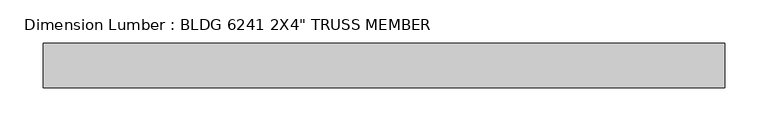
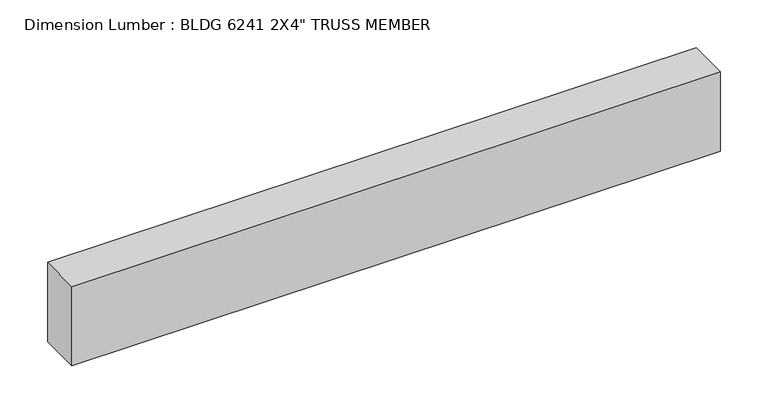
"""IFC4 building model written with IfcOpenShell, lengths in millimetres: beam geometry."""

import ifcopenshell
import ifcopenshell.guid

model = None  # the IFC model being written
_history = None  # IfcOwnerHistory: only IFC2X3 demands one
_inside = {}  # id of a spatial element -> (the spatial element, [elements in it])
_under = {}  # id of a project, library or spatial element -> (it, [spatial elements below it])
_declared = {}  # id of a project -> (the project, [libraries it declares])
_typed = {}  # id of a type object -> (the type object, [elements of that type])
_made_of = {}  # id of a material, layer set ... -> (it, [elements and type objects made of it])


def new_model(schema):
    """Start an empty IFC model of exactly this schema.

    Asked for "IFC4X3", IfcOpenShell would pick the latest addendum, in which some entities
    have other attributes; the version numbers below select the first issue.
    IFC2X3 requires an IfcOwnerHistory on every rooted entity: one is made here for all.
    """
    global model, _history
    if schema == "IFC4X3":
        model = ifcopenshell.file(schema_version=(4, 3, 0, 0))
    else:
        model = ifcopenshell.file(schema=schema)
    _inside.clear()
    _under.clear()
    _declared.clear()
    _typed.clear()
    _made_of.clear()
    _history = None
    if model.schema == "IFC2X3":
        org = make("IfcOrganization", Name="unknown")
        user = make(
            "IfcPersonAndOrganization",
            ThePerson=make("IfcPerson", FamilyName="unknown"),
            TheOrganization=org,
        )
        app = make(
            "IfcApplication",
            ApplicationDeveloper=org,
            Version="unknown",
            ApplicationFullName="unknown",
            ApplicationIdentifier="unknown",
        )
        _history = make(
            "IfcOwnerHistory",
            OwningUser=user,
            OwningApplication=app,
            ChangeAction="ADDED",
            CreationDate=0,
        )
    return model


def make(cls, **values):
    """One entity of the class cls with the attributes given. An attribute that is None is left unset."""
    return model.create_entity(
        cls, **{name: value for name, value in values.items() if value is not None}
    )


def rooted(cls, **values):
    """An entity with a GlobalId (a new one), such as an element, a storey or a relation."""
    return make(cls, GlobalId=ifcopenshell.guid.new(), OwnerHistory=_history, **values)


def si_unit(unit_type, name, prefix=None):
    """IfcSIUnit, for example si_unit("LENGTHUNIT", "METRE", prefix="MILLI")."""
    return make("IfcSIUnit", UnitType=unit_type, Prefix=prefix, Name=name)


def assignment(units):
    """IfcUnitAssignment: the units of a project."""
    return None if units is None else make("IfcUnitAssignment", Units=units)


def point(xyz):
    """IfcCartesianPoint."""
    return None if xyz is None else make("IfcCartesianPoint", Coordinates=xyz)


def direction(xyz):
    """IfcDirection."""
    return None if xyz is None else make("IfcDirection", DirectionRatios=xyz)


def frame(location, z_axis=None, x_axis=None):
    """IfcAxis2Placement3D, a coordinate frame: its origin and axes. An axis left out is left unset."""
    return make(
        "IfcAxis2Placement3D",
        Location=point(location),
        Axis=direction(z_axis),
        RefDirection=direction(x_axis),
    )


def origin():
    """The frame at (0, 0, 0) with its axes left unset."""
    return frame((0.0, 0.0, 0.0))


def place(relative_to, where):
    """IfcLocalPlacement: puts the frame where relative to a parent placement (None: the world)."""
    return make(
        "IfcLocalPlacement", PlacementRelTo=relative_to, RelativePlacement=where
    )


def context(
    kind, dimensions, precision=None, world=None, true_north=None, identifier=None
):
    """IfcGeometricRepresentationContext, for example the 3D "Model" context."""
    return make(
        "IfcGeometricRepresentationContext",
        ContextIdentifier=identifier,
        ContextType=kind,
        CoordinateSpaceDimension=dimensions,
        Precision=precision,
        WorldCoordinateSystem=world,
        TrueNorth=true_north,
    )


def project(units=None, contexts=None):
    """IfcProject with its units and contexts."""
    return rooted(
        "IfcProject",
        Name="project",
        RepresentationContexts=contexts,
        UnitsInContext=assignment(units),
    )


def spatial(cls, under=None, at=None, **own):
    """A site, building, storey or space (cls), placed at a placement, below another one or the project."""
    s = rooted(cls, ObjectPlacement=at, **own)
    if under is not None:
        _under.setdefault(under.id(), (under, []))[1].append(s)
    return s


def polyline(points):
    """IfcPolyline through the points."""
    return make("IfcPolyline", Points=[point(p) for p in points])


def outline(outer, holes=None, kind="AREA"):
    """IfcArbitraryClosedProfileDef: a profile drawn as a closed curve; with holes, ...WithVoids."""
    if holes is None:
        return make("IfcArbitraryClosedProfileDef", ProfileType=kind, OuterCurve=outer)
    return make(
        "IfcArbitraryProfileDefWithVoids",
        ProfileType=kind,
        OuterCurve=outer,
        InnerCurves=holes,
    )


def extrude(swept, where, along, depth):
    """IfcExtrudedAreaSolid: the profile swept, set in the frame where, extruded along a direction by depth."""
    return make(
        "IfcExtrudedAreaSolid",
        SweptArea=swept,
        Position=where,
        ExtrudedDirection=direction(along),
        Depth=depth,
    )


def shape(context_of_items, identifier, shape_type, items):
    """IfcShapeRepresentation: the items that make up one representation, for example the "Body"."""
    return make(
        "IfcShapeRepresentation",
        ContextOfItems=context_of_items,
        RepresentationIdentifier=identifier,
        RepresentationType=shape_type,
        Items=items,
    )


def source(mapping_origin, context_of_items, identifier, shape_type, items):
    """IfcRepresentationMap: a shape defined once, which mapped items show again and again."""
    return make(
        "IfcRepresentationMap",
        MappingOrigin=mapping_origin,
        MappedRepresentation=shape(context_of_items, identifier, shape_type, items),
    )


def transform(
    local_origin,
    x_axis=None,
    y_axis=None,
    z_axis=None,
    scale=None,
    scale2=None,
    scale3=None,
    uniform=True,
):
    """IfcCartesianTransformationOperator3D, or its non-uniform kind. x_axis, y_axis, z_axis: its Axis1, 2, 3."""
    if uniform:
        return make(
            "IfcCartesianTransformationOperator3D",
            Axis1=direction(x_axis),
            Axis2=direction(y_axis),
            LocalOrigin=point(local_origin),
            Scale=scale,
            Axis3=direction(z_axis),
        )
    return make(
        "IfcCartesianTransformationOperator3DnonUniform",
        Axis1=direction(x_axis),
        Axis2=direction(y_axis),
        LocalOrigin=point(local_origin),
        Scale=scale,
        Axis3=direction(z_axis),
        Scale2=scale2,
        Scale3=scale3,
    )


def mapped(mapping_source, mapping_target):
    """IfcMappedItem: shows the shape of a source again, moved by a transform."""
    return make(
        "IfcMappedItem", MappingSource=mapping_source, MappingTarget=mapping_target
    )


def made_of(thing, what):
    """Note that an element or type object is made of a material, layer set ...; save() writes the relation."""
    if what is not None:
        _made_of.setdefault(what.id(), (what, []))[1].append(thing)
    return thing


def element(
    cls,
    number,
    at=None,
    inside=None,
    cuts=None,
    type_object=None,
    material=None,
    context=None,
    identifier="Body",
    shape_type=None,
    held_by="IfcProductDefinitionShape",
    body=None,
    shapes=None,
    **own,
):
    """One element of the class cls, such as IfcWall. Its Tag is "e" and its number.

    at: its placement. inside: the storey or other place that contains it. cuts: it is an
    opening in that element (IfcRelVoidsElement). A single representation is given by context,
    identifier, shape_type and body (its items); several are given by shapes. held_by: the class
    of the entity that holds the representations. save() writes the other relations.
    """
    e = rooted(cls, Tag="e%d" % number, ObjectPlacement=at, **own)
    if body is not None:
        shapes = [shape(context, identifier, shape_type, body)]
    if shapes is not None:
        e.Representation = make(held_by, Representations=shapes)
    if inside is not None:
        _inside.setdefault(inside.id(), (inside, []))[1].append(e)
    if cuts is not None:
        rooted(
            "IfcRelVoidsElement", RelatingBuildingElement=cuts, RelatedOpeningElement=e
        )
    if type_object is not None:
        _typed.setdefault(type_object.id(), (type_object, []))[1].append(e)
    return made_of(e, material)


def aggregate(whole, parts):
    """IfcRelAggregates: a whole, such as a stair, and the parts it consists of."""
    return rooted("IfcRelAggregates", RelatingObject=whole, RelatedObjects=parts)


def save(model, path):
    """Write the relations noted so far, then the file.

    IfcRelAggregates (storeys below a building ...), IfcRelContainedInSpatialStructure (elements
    in a storey), IfcRelDefinesByType, IfcRelAssociatesMaterial and IfcRelDeclares: one each for
    every whole, place, type object, material and project.
    """
    for whole, parts in _under.values():
        aggregate(whole, parts)
    for where, things in _inside.values():
        rooted(
            "IfcRelContainedInSpatialStructure",
            RelatedElements=things,
            RelatingStructure=where,
        )
    for kind, things in _typed.values():
        rooted("IfcRelDefinesByType", RelatedObjects=things, RelatingType=kind)
    for what, things in _made_of.values():
        rooted("IfcRelAssociatesMaterial", RelatedObjects=things, RelatingMaterial=what)
    for by, libraries in _declared.values():
        rooted("IfcRelDeclares", RelatingContext=by, RelatedDefinitions=libraries)
    model.write(path)


def beam_ce158ae4(model_context):
    return source(origin(), model_context, "Body", "SweptSolid", [
        extrude(outline(polyline([(392.1124994, 25.4), (392.1124994, -25.4), (-392.1125, -25.4), (-392.1125, 25.4), (392.1124994, 25.4)])), frame((0.0, 0.0, -50.8), z_axis=(0.0, 0.0, 1.0), x_axis=(1.0, 0.0, 0.0)), (0.0, 0.0, 1.0), 101.6),
    ])


if __name__ == "__main__":
    model = new_model("IFC4")
    model_context = context("Model", 3, world=origin())
    ifc_project = project(units=[si_unit("LENGTHUNIT", "METRE", prefix="MILLI")], contexts=[model_context])
    site = spatial("IfcSite", under=ifc_project)
    building = spatial("IfcBuilding", under=site)
    placement = place(None, origin())
    beam_shape = beam_ce158ae4(model_context)
    element("IfcBeam", 1, ObjectType="Dimension Lumber : BLDG 6241 2X4\" TRUSS MEMBER", at=placement, inside=building, context=model_context, shape_type="MappedRepresentation", body=[
        mapped(beam_shape, transform((0.0, 0.0, 0.0), x_axis=(1.0, 0.0, 0.0), y_axis=(0.0, 1.0, 0.0), z_axis=(0.0, 0.0, 1.0))),
    ])
    save(model, "model.ifc")

# Revit data of these elements
# Type "Dimension Lumber : BLDG 6241 2X4\" TRUSS MEMBER"
#   Assembly Code = "B10"
#   A = 0.273472 SF
#   Length [instance default] = 5' - 0"
#   b = 0' - 2"
#   d = 0' - 4"
#   Structural Material [instance default] = Softwood, Lumber
# Element 1 (IfcBeam, "Dimension Lumber : BLDG 6241 2X4\" TRUSS MEMBER")
#   Materials on its faces: "Softwood, Lumber"
# Materials
#   "Softwood, Lumber": class "Wood", colour RGB 223 192 134, transparency 0, Description = "Pinus Echinata", Cost = 0
